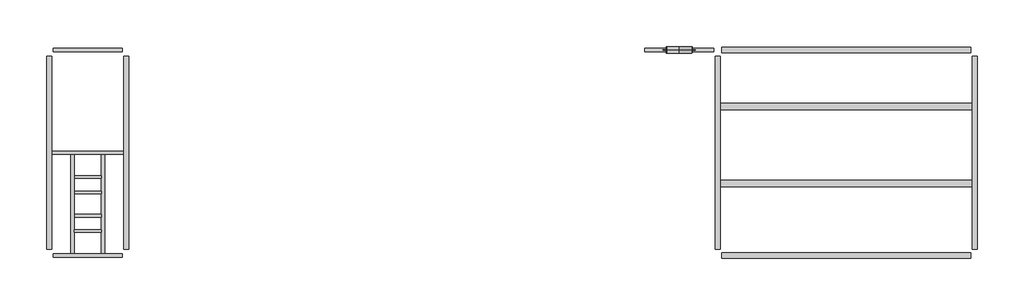
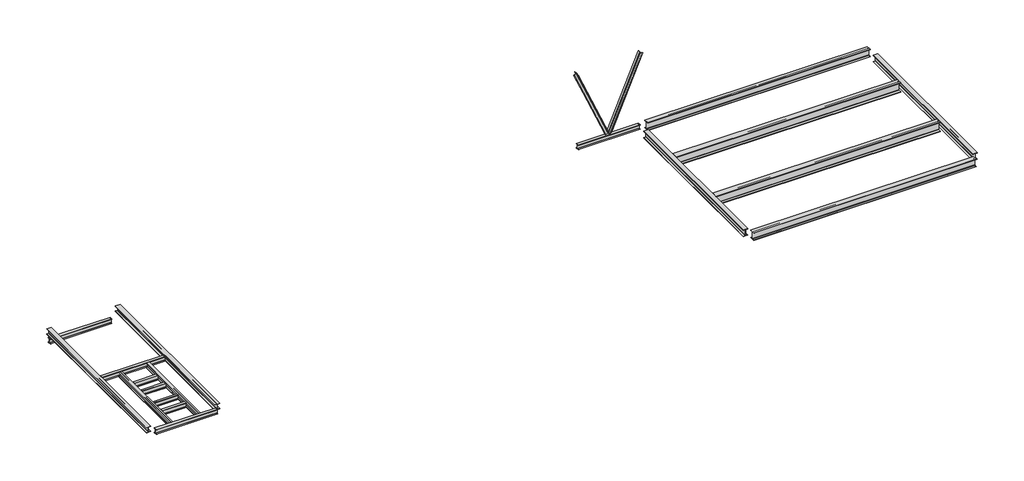
# One storey: 20 beams.
"""IFC4 building model written with IfcOpenShell, lengths in millimetres."""

import ifcopenshell
import ifcopenshell.guid

model = None  # the IFC model being written
_history = None  # IfcOwnerHistory: only IFC2X3 demands one
_inside = {}  # id of a spatial element -> (the spatial element, [elements in it])
_under = {}  # id of a project, library or spatial element -> (it, [spatial elements below it])
_declared = {}  # id of a project -> (the project, [libraries it declares])
_typed = {}  # id of a type object -> (the type object, [elements of that type])
_made_of = {}  # id of a material, layer set ... -> (it, [elements and type objects made of it])


def new_model(schema):
    """Start an empty IFC model of exactly this schema.

    Asked for "IFC4X3", IfcOpenShell would pick the latest addendum, in which some entities
    have other attributes; the version numbers below select the first issue.
    IFC2X3 requires an IfcOwnerHistory on every rooted entity: one is made here for all.
    """
    global model, _history
    if schema == "IFC4X3":
        model = ifcopenshell.file(schema_version=(4, 3, 0, 0))
    else:
        model = ifcopenshell.file(schema=schema)
    _inside.clear()
    _under.clear()
    _declared.clear()
    _typed.clear()
    _made_of.clear()
    _history = None
    if model.schema == "IFC2X3":
        org = make("IfcOrganization", Name="unknown")
        user = make(
            "IfcPersonAndOrganization",
            ThePerson=make("IfcPerson", FamilyName="unknown"),
            TheOrganization=org,
        )
        app = make(
            "IfcApplication",
            ApplicationDeveloper=org,
            Version="unknown",
            ApplicationFullName="unknown",
            ApplicationIdentifier="unknown",
        )
        _history = make(
            "IfcOwnerHistory",
            OwningUser=user,
            OwningApplication=app,
            ChangeAction="ADDED",
            CreationDate=0,
        )
    return model


def make(cls, **values):
    """One entity of the class cls with the attributes given. An attribute that is None is left unset."""
    return model.create_entity(
        cls, **{name: value for name, value in values.items() if value is not None}
    )


def rooted(cls, **values):
    """An entity with a GlobalId (a new one), such as an element, a storey or a relation."""
    return make(cls, GlobalId=ifcopenshell.guid.new(), OwnerHistory=_history, **values)


def si_unit(unit_type, name, prefix=None):
    """IfcSIUnit, for example si_unit("LENGTHUNIT", "METRE", prefix="MILLI")."""
    return make("IfcSIUnit", UnitType=unit_type, Prefix=prefix, Name=name)


def assignment(units):
    """IfcUnitAssignment: the units of a project."""
    return None if units is None else make("IfcUnitAssignment", Units=units)


def point(xyz):
    """IfcCartesianPoint."""
    return None if xyz is None else make("IfcCartesianPoint", Coordinates=xyz)


def direction(xyz):
    """IfcDirection."""
    return None if xyz is None else make("IfcDirection", DirectionRatios=xyz)


def frame(location, z_axis=None, x_axis=None):
    """IfcAxis2Placement3D, a coordinate frame: its origin and axes. An axis left out is left unset."""
    return make(
        "IfcAxis2Placement3D",
        Location=point(location),
        Axis=direction(z_axis),
        RefDirection=direction(x_axis),
    )


def frame_2d(location, x_axis=None):
    """IfcAxis2Placement2D, a coordinate frame in the plane: its origin and x axis."""
    return make(
        "IfcAxis2Placement2D", Location=point(location), RefDirection=direction(x_axis)
    )


def origin():
    """The frame at (0, 0, 0) with its axes left unset."""
    return frame((0.0, 0.0, 0.0))


def place(relative_to, where):
    """IfcLocalPlacement: puts the frame where relative to a parent placement (None: the world)."""
    return make(
        "IfcLocalPlacement", PlacementRelTo=relative_to, RelativePlacement=where
    )


def context(
    kind, dimensions, precision=None, world=None, true_north=None, identifier=None
):
    """IfcGeometricRepresentationContext, for example the 3D "Model" context."""
    return make(
        "IfcGeometricRepresentationContext",
        ContextIdentifier=identifier,
        ContextType=kind,
        CoordinateSpaceDimension=dimensions,
        Precision=precision,
        WorldCoordinateSystem=world,
        TrueNorth=true_north,
    )


def project(units=None, contexts=None):
    """IfcProject with its units and contexts."""
    return rooted(
        "IfcProject",
        Name="project",
        RepresentationContexts=contexts,
        UnitsInContext=assignment(units),
    )


def spatial(cls, under=None, at=None, **own):
    """A site, building, storey or space (cls), placed at a placement, below another one or the project."""
    s = rooted(cls, ObjectPlacement=at, **own)
    if under is not None:
        _under.setdefault(under.id(), (under, []))[1].append(s)
    return s


def polyline(points):
    """IfcPolyline through the points."""
    return make("IfcPolyline", Points=[point(p) for p in points])


def circle_curve(where, radius):
    """IfcCircle in the frame where."""
    return make("IfcCircle", Position=where, Radius=radius)


def trimmed(basis, trim1, trim2, sense, master):
    """IfcTrimmedCurve: the piece of a basis curve between two trims."""
    return make(
        "IfcTrimmedCurve",
        BasisCurve=basis,
        Trim1=trim1,
        Trim2=trim2,
        SenseAgreement=sense,
        MasterRepresentation=master,
    )


def segment(curve, same_sense, transition):
    """IfcCompositeCurveSegment."""
    return make(
        "IfcCompositeCurveSegment",
        Transition=transition,
        SameSense=same_sense,
        ParentCurve=curve,
    )


def composite_curve(segments, self_intersect=None):
    """IfcCompositeCurve: segments joined end to end."""
    return make("IfcCompositeCurve", Segments=segments, SelfIntersect=self_intersect)


def outline(outer, holes=None, kind="AREA"):
    """IfcArbitraryClosedProfileDef: a profile drawn as a closed curve; with holes, ...WithVoids."""
    if holes is None:
        return make("IfcArbitraryClosedProfileDef", ProfileType=kind, OuterCurve=outer)
    return make(
        "IfcArbitraryProfileDefWithVoids",
        ProfileType=kind,
        OuterCurve=outer,
        InnerCurves=holes,
    )


def extrude(swept, where, along, depth):
    """IfcExtrudedAreaSolid: the profile swept, set in the frame where, extruded along a direction by depth."""
    return make(
        "IfcExtrudedAreaSolid",
        SweptArea=swept,
        Position=where,
        ExtrudedDirection=direction(along),
        Depth=depth,
    )


def shape(context_of_items, identifier, shape_type, items):
    """IfcShapeRepresentation: the items that make up one representation, for example the "Body"."""
    return make(
        "IfcShapeRepresentation",
        ContextOfItems=context_of_items,
        RepresentationIdentifier=identifier,
        RepresentationType=shape_type,
        Items=items,
    )


def source(mapping_origin, context_of_items, identifier, shape_type, items):
    """IfcRepresentationMap: a shape defined once, which mapped items show again and again."""
    return make(
        "IfcRepresentationMap",
        MappingOrigin=mapping_origin,
        MappedRepresentation=shape(context_of_items, identifier, shape_type, items),
    )


def transform(
    local_origin,
    x_axis=None,
    y_axis=None,
    z_axis=None,
    scale=None,
    scale2=None,
    scale3=None,
    uniform=True,
):
    """IfcCartesianTransformationOperator3D, or its non-uniform kind. x_axis, y_axis, z_axis: its Axis1, 2, 3."""
    if uniform:
        return make(
            "IfcCartesianTransformationOperator3D",
            Axis1=direction(x_axis),
            Axis2=direction(y_axis),
            LocalOrigin=point(local_origin),
            Scale=scale,
            Axis3=direction(z_axis),
        )
    return make(
        "IfcCartesianTransformationOperator3DnonUniform",
        Axis1=direction(x_axis),
        Axis2=direction(y_axis),
        LocalOrigin=point(local_origin),
        Scale=scale,
        Axis3=direction(z_axis),
        Scale2=scale2,
        Scale3=scale3,
    )


def mapped(mapping_source, mapping_target):
    """IfcMappedItem: shows the shape of a source again, moved by a transform."""
    return make(
        "IfcMappedItem", MappingSource=mapping_source, MappingTarget=mapping_target
    )


def made_of(thing, what):
    """Note that an element or type object is made of a material, layer set ...; save() writes the relation."""
    if what is not None:
        _made_of.setdefault(what.id(), (what, []))[1].append(thing)
    return thing


def element(
    cls,
    number,
    at=None,
    inside=None,
    cuts=None,
    type_object=None,
    material=None,
    context=None,
    identifier="Body",
    shape_type=None,
    held_by="IfcProductDefinitionShape",
    body=None,
    shapes=None,
    **own,
):
    """One element of the class cls, such as IfcWall. Its Tag is "e" and its number.

    at: its placement. inside: the storey or other place that contains it. cuts: it is an
    opening in that element (IfcRelVoidsElement). A single representation is given by context,
    identifier, shape_type and body (its items); several are given by shapes. held_by: the class
    of the entity that holds the representations. save() writes the other relations.
    """
    e = rooted(cls, Tag="e%d" % number, ObjectPlacement=at, **own)
    if body is not None:
        shapes = [shape(context, identifier, shape_type, body)]
    if shapes is not None:
        e.Representation = make(held_by, Representations=shapes)
    if inside is not None:
        _inside.setdefault(inside.id(), (inside, []))[1].append(e)
    if cuts is not None:
        rooted(
            "IfcRelVoidsElement", RelatingBuildingElement=cuts, RelatedOpeningElement=e
        )
    if type_object is not None:
        _typed.setdefault(type_object.id(), (type_object, []))[1].append(e)
    return made_of(e, material)


def aggregate(whole, parts):
    """IfcRelAggregates: a whole, such as a stair, and the parts it consists of."""
    return rooted("IfcRelAggregates", RelatingObject=whole, RelatedObjects=parts)


def save(model, path):
    """Write the relations noted so far, then the file.

    IfcRelAggregates (storeys below a building ...), IfcRelContainedInSpatialStructure (elements
    in a storey), IfcRelDefinesByType, IfcRelAssociatesMaterial and IfcRelDeclares: one each for
    every whole, place, type object, material and project.
    """
    for whole, parts in _under.values():
        aggregate(whole, parts)
    for where, things in _inside.values():
        rooted(
            "IfcRelContainedInSpatialStructure",
            RelatedElements=things,
            RelatingStructure=where,
        )
    for kind, things in _typed.values():
        rooted("IfcRelDefinesByType", RelatedObjects=things, RelatingType=kind)
    for what, things in _made_of.values():
        rooted("IfcRelAssociatesMaterial", RelatedObjects=things, RelatingMaterial=what)
    for by, libraries in _declared.values():
        rooted("IfcRelDeclares", RelatingContext=by, RelatedDefinitions=libraries)
    model.write(path)


def beam_96e87236(model_context):
    return source(origin(), model_context, "Body", "SweptSolid", [
        extrude(outline(composite_curve([segment(polyline([(0.0, 36.4), (130.0, 36.4)]), True, "CONTINUOUS"), segment(trimmed(circle_curve(frame_2d((118.0, 36.4)), 12.0), [point((130.0, 36.4))], [point((118.0, 24.4))], False, "CARTESIAN"), True, "CONTINUOUS"), segment(polyline([(118.0, 24.4), (24.0, 24.4)]), True, "CONTINUOUS"), segment(trimmed(circle_curve(frame_2d((24.0, 12.4)), 12.0), [point((24.0, 24.4))], [point((12.0, 12.4))], True, "CARTESIAN"), True, "CONTINUOUS"), segment(polyline([(12.0, 12.4), (12.0, -81.6)]), True, "CONTINUOUS"), segment(trimmed(circle_curve(frame_2d((0.0, -81.6)), 12.0), [point((12.0, -81.6))], [point((0.0, -93.6))], False, "CARTESIAN"), True, "CONTINUOUS"), segment(polyline([(0.0, -93.6), (0.0, 36.4)]), True, "CONTINUOUS")], self_intersect=False)), frame((-1749.149537, 0.0, 0.0), z_axis=(1.0, 0.0, 0.0), x_axis=(0.0, 1.0, 0.0)), (0.0, 0.0, 1.0), 3498.299074),
        extrude(outline(composite_curve([segment(polyline([(0.0, 36.4), (0.0, -93.6)]), True, "CONTINUOUS"), segment(trimmed(circle_curve(frame_2d((0.0, -81.6)), 12.0), [point((0.0, -93.6))], [point((-12.0, -81.6))], False, "CARTESIAN"), True, "CONTINUOUS"), segment(polyline([(-12.0, -81.6), (-12.0, 12.4)]), True, "CONTINUOUS"), segment(trimmed(circle_curve(frame_2d((-24.0, 12.4)), 12.0), [point((-12.0, 12.4))], [point((-24.0, 24.4))], True, "CARTESIAN"), True, "CONTINUOUS"), segment(polyline([(-24.0, 24.4), (-118.0, 24.4)]), True, "CONTINUOUS"), segment(trimmed(circle_curve(frame_2d((-118.0, 36.4)), 12.0), [point((-118.0, 24.4))], [point((-130.0, 36.4))], False, "CARTESIAN"), True, "CONTINUOUS"), segment(polyline([(-130.0, 36.4), (0.0, 36.4)]), True, "CONTINUOUS")], self_intersect=False)), frame((-1749.149537, 0.0, 0.0), z_axis=(1.0, 0.0, 0.0), x_axis=(0.0, 1.0, 0.0)), (0.0, 0.0, 1.0), 3498.299074),
    ])


def steel_framing_w_astm_a6m_f33feb28(model_context):
    return source(origin(), model_context, "Body", "SweptSolid", [
        extrude(outline(composite_curve([segment(polyline([(67.0, -94.8), (67.0, -105.0), (-67.0, -105.0), (-67.0, -94.8), (-10.775, -94.8)]), True, "CONTINUOUS"), segment(trimmed(circle_curve(frame_2d((-10.775, -87.2)), 7.6), [point((-10.775, -94.8))], [point((-3.175, -87.2))], True, "CARTESIAN"), True, "CONTINUOUS"), segment(polyline([(-3.175, -87.2), (-3.175, 87.2)]), True, "CONTINUOUS"), segment(trimmed(circle_curve(frame_2d((-10.775, 87.2)), 7.6), [point((-3.175, 87.2))], [point((-10.775, 94.8))], True, "CARTESIAN"), True, "CONTINUOUS"), segment(polyline([(-10.775, 94.8), (-67.0, 94.8), (-67.0, 105.0), (67.0, 105.0), (67.0, 94.8), (10.775, 94.8)]), True, "CONTINUOUS"), segment(trimmed(circle_curve(frame_2d((10.775, 87.2)), 7.6), [point((10.775, 94.8))], [point((3.175, 87.2))], True, "CARTESIAN"), True, "CONTINUOUS"), segment(polyline([(3.175, 87.2), (3.175, -87.2)]), True, "CONTINUOUS"), segment(trimmed(circle_curve(frame_2d((10.775, -87.2)), 7.6), [point((3.175, -87.2))], [point((10.775, -94.8))], True, "CARTESIAN"), True, "CONTINUOUS"), segment(polyline([(10.775, -94.8), (67.0, -94.8)]), True, "CONTINUOUS")], self_intersect=False)), frame((-1346.3, 0.0, 0.0), z_axis=(1.0, 0.0, 0.0), x_axis=(0.0, 1.0, 0.0)), (0.0, 0.0, 1.0), 2692.6),
    ])


def steel_framing_w_astm_a6m_fe1e75f4(model_context):
    return source(origin(), model_context, "Body", "SweptSolid", [
        extrude(outline(composite_curve([segment(polyline([(67.0, -94.8), (67.0, -105.0), (-67.0, -105.0), (-67.0, -94.8), (-10.775, -94.8)]), True, "CONTINUOUS"), segment(trimmed(circle_curve(frame_2d((-10.775, -87.2)), 7.6), [point((-10.775, -94.8))], [point((-3.175, -87.2))], True, "CARTESIAN"), True, "CONTINUOUS"), segment(polyline([(-3.175, -87.2), (-3.175, 87.2)]), True, "CONTINUOUS"), segment(trimmed(circle_curve(frame_2d((-10.775, 87.2)), 7.6), [point((-3.175, 87.2))], [point((-10.775, 94.8))], True, "CARTESIAN"), True, "CONTINUOUS"), segment(polyline([(-10.775, 94.8), (-67.0, 94.8), (-67.0, 105.0), (67.0, 105.0), (67.0, 94.8), (10.775, 94.8)]), True, "CONTINUOUS"), segment(trimmed(circle_curve(frame_2d((10.775, 87.2)), 7.6), [point((10.775, 94.8))], [point((3.175, 87.2))], True, "CARTESIAN"), True, "CONTINUOUS"), segment(polyline([(3.175, 87.2), (3.175, -87.2)]), True, "CONTINUOUS"), segment(trimmed(circle_curve(frame_2d((10.775, -87.2)), 7.6), [point((3.175, -87.2))], [point((10.775, -94.8))], True, "CARTESIAN"), True, "CONTINUOUS"), segment(polyline([(10.775, -94.8), (67.0, -94.8)]), True, "CONTINUOUS")], self_intersect=False)), frame((-1386.3, 0.0, 0.0), z_axis=(1.0, 0.0, 0.0), x_axis=(0.0, 1.0, 0.0)), (0.0, 0.0, 1.0), 2772.6),
    ])


def steel_framing_w_astm_a6m_8cea9429(model_context):
    return source(origin(), model_context, "Body", "SweptSolid", [
        extrude(outline(composite_curve([segment(polyline([(101.5, -137.9), (101.5, -151.0), (-101.5, -151.0), (-101.5, -137.9), (-16.545, -137.9)]), True, "CONTINUOUS"), segment(trimmed(circle_curve(frame_2d((-16.545, -125.1)), 12.8), [point((-16.545, -137.9))], [point((-3.745, -125.1))], True, "CARTESIAN"), True, "CONTINUOUS"), segment(polyline([(-3.745, -125.1), (-3.745, 125.1)]), True, "CONTINUOUS"), segment(trimmed(circle_curve(frame_2d((-16.545, 125.1)), 12.8), [point((-3.745, 125.1))], [point((-16.545, 137.9))], True, "CARTESIAN"), True, "CONTINUOUS"), segment(polyline([(-16.545, 137.9), (-101.5, 137.9), (-101.5, 151.0), (101.5, 151.0), (101.5, 137.9), (16.545, 137.9)]), True, "CONTINUOUS"), segment(trimmed(circle_curve(frame_2d((16.545, 125.1)), 12.8), [point((16.545, 137.9))], [point((3.745, 125.1))], True, "CARTESIAN"), True, "CONTINUOUS"), segment(polyline([(3.745, 125.1), (3.745, -125.1)]), True, "CONTINUOUS"), segment(trimmed(circle_curve(frame_2d((16.545, -125.1)), 12.8), [point((3.745, -125.1))], [point((16.545, -137.9))], True, "CARTESIAN"), True, "CONTINUOUS"), segment(polyline([(16.545, -137.9), (101.5, -137.9)]), True, "CONTINUOUS")], self_intersect=False)), frame((-3753.8, 0.0, 0.0), z_axis=(1.0, 0.0, 0.0), x_axis=(0.0, 1.0, 0.0)), (0.0, 0.0, 1.0), 7507.6),
    ])


def steel_framing_w_astm_a6m_fd2852ff(model_context):
    return source(origin(), model_context, "Body", "SweptSolid", [
        extrude(outline(composite_curve([segment(polyline([(67.0, -94.8), (67.0, -105.0), (-67.0, -105.0), (-67.0, -94.8), (-10.775, -94.8)]), True, "CONTINUOUS"), segment(trimmed(circle_curve(frame_2d((-10.775, -87.2)), 7.6), [point((-10.775, -94.8))], [point((-3.175, -87.2))], True, "CARTESIAN"), True, "CONTINUOUS"), segment(polyline([(-3.175, -87.2), (-3.175, 87.2)]), True, "CONTINUOUS"), segment(trimmed(circle_curve(frame_2d((-10.775, 87.2)), 7.6), [point((-3.175, 87.2))], [point((-10.775, 94.8))], True, "CARTESIAN"), True, "CONTINUOUS"), segment(polyline([(-10.775, 94.8), (-67.0, 94.8), (-67.0, 105.0), (67.0, 105.0), (67.0, 94.8), (10.775, 94.8)]), True, "CONTINUOUS"), segment(trimmed(circle_curve(frame_2d((10.775, 87.2)), 7.6), [point((10.775, 94.8))], [point((3.175, 87.2))], True, "CARTESIAN"), True, "CONTINUOUS"), segment(polyline([(3.175, 87.2), (3.175, -87.2)]), True, "CONTINUOUS"), segment(trimmed(circle_curve(frame_2d((10.775, -87.2)), 7.6), [point((3.175, -87.2))], [point((10.775, -94.8))], True, "CARTESIAN"), True, "CONTINUOUS"), segment(polyline([(10.775, -94.8), (67.0, -94.8)]), True, "CONTINUOUS")], self_intersect=False)), frame((-1920.3, 0.0, 0.0), z_axis=(1.0, 0.0, 0.0), x_axis=(0.0, 1.0, 0.0)), (0.0, 0.0, 1.0), 3840.6),
    ])


def steel_framing_w_astm_a6m_80da07c9(model_context):
    return source(origin(), model_context, "Body", "SweptSolid", [
        extrude(outline(composite_curve([segment(polyline([(101.0, -112.5), (101.0, -123.5), (-101.0, -123.5), (-101.0, -112.5), (-16.385, -112.5)]), True, "CONTINUOUS"), segment(trimmed(circle_curve(frame_2d((-16.385, -99.8)), 12.7), [point((-16.385, -112.5))], [point((-3.685, -99.8))], True, "CARTESIAN"), True, "CONTINUOUS"), segment(polyline([(-3.685, -99.8), (-3.685, 99.8)]), True, "CONTINUOUS"), segment(trimmed(circle_curve(frame_2d((-16.385, 99.8)), 12.7), [point((-3.685, 99.8))], [point((-16.385, 112.5))], True, "CARTESIAN"), True, "CONTINUOUS"), segment(polyline([(-16.385, 112.5), (-101.0, 112.5), (-101.0, 123.5), (101.0, 123.5), (101.0, 112.5), (16.385, 112.5)]), True, "CONTINUOUS"), segment(trimmed(circle_curve(frame_2d((16.385, 99.8)), 12.7), [point((16.385, 112.5))], [point((3.685, 99.8))], True, "CARTESIAN"), True, "CONTINUOUS"), segment(polyline([(3.685, 99.8), (3.685, -99.8)]), True, "CONTINUOUS"), segment(trimmed(circle_curve(frame_2d((16.385, -99.8)), 12.7), [point((3.685, -99.8))], [point((16.385, -112.5))], True, "CARTESIAN"), True, "CONTINUOUS"), segment(polyline([(16.385, -112.5), (101.0, -112.5)]), True, "CONTINUOUS")], self_intersect=False)), frame((-3753.8, 0.0, 0.0), z_axis=(1.0, 0.0, 0.0), x_axis=(0.0, 1.0, 0.0)), (0.0, 0.0, 1.0), 7507.6),
    ])


def steel_framing_w_astm_a6m_d888c6d0(model_context):
    return source(origin(), model_context, "Body", "SweptSolid", [
        extrude(outline(composite_curve([segment(polyline([(102.5, -159.7), (102.5, -176.5), (-102.5, -176.5), (-102.5, -159.7), (-19.7, -159.7)]), True, "CONTINUOUS"), segment(trimmed(circle_curve(frame_2d((-19.7, -144.7)), 15.0), [point((-19.7, -159.7))], [point((-4.7, -144.7))], True, "CARTESIAN"), True, "CONTINUOUS"), segment(polyline([(-4.7, -144.7), (-4.7, 144.7)]), True, "CONTINUOUS"), segment(trimmed(circle_curve(frame_2d((-19.7, 144.7)), 15.0), [point((-4.7, 144.7))], [point((-19.7, 159.7))], True, "CARTESIAN"), True, "CONTINUOUS"), segment(polyline([(-19.7, 159.7), (-102.5, 159.7), (-102.5, 176.5), (102.5, 176.5), (102.5, 159.7), (19.7, 159.7)]), True, "CONTINUOUS"), segment(trimmed(circle_curve(frame_2d((19.7, 144.7)), 15.0), [point((19.7, 159.7))], [point((4.7, 144.7))], True, "CARTESIAN"), True, "CONTINUOUS"), segment(polyline([(4.7, 144.7), (4.7, -144.7)]), True, "CONTINUOUS"), segment(trimmed(circle_curve(frame_2d((19.7, -144.7)), 15.0), [point((4.7, -144.7))], [point((19.7, -159.7))], True, "CARTESIAN"), True, "CONTINUOUS"), segment(polyline([(19.7, -159.7), (102.5, -159.7)]), True, "CONTINUOUS")], self_intersect=False)), frame((-4846.3, 0.0, 0.0), z_axis=(1.0, 0.0, 0.0), x_axis=(0.0, 1.0, 0.0)), (0.0, 0.0, 1.0), 9692.6),
    ])


def steel_framing_w_astm_a6m_4c16a149(model_context):
    return source(origin(), model_context, "Body", "SweptSolid", [
        extrude(outline(composite_curve([segment(polyline([(131.0, -190.2), (131.0, -209.5), (-131.0, -209.5), (-131.0, -190.2), (-16.0, -190.2)]), True, "CONTINUOUS"), segment(trimmed(circle_curve(frame_2d((-16.0, -180.0)), 10.2), [point((-16.0, -190.2))], [point((-5.8, -180.0))], True, "CARTESIAN"), True, "CONTINUOUS"), segment(polyline([(-5.8, -180.0), (-5.8, 180.0)]), True, "CONTINUOUS"), segment(trimmed(circle_curve(frame_2d((-16.0, 180.0)), 10.2), [point((-5.8, 180.0))], [point((-16.0, 190.2))], True, "CARTESIAN"), True, "CONTINUOUS"), segment(polyline([(-16.0, 190.2), (-131.0, 190.2), (-131.0, 209.5), (131.0, 209.5), (131.0, 190.2), (16.0, 190.2)]), True, "CONTINUOUS"), segment(trimmed(circle_curve(frame_2d((16.0, 180.0)), 10.2), [point((16.0, 190.2))], [point((5.8, 180.0))], True, "CARTESIAN"), True, "CONTINUOUS"), segment(polyline([(5.8, 180.0), (5.8, -180.0)]), True, "CONTINUOUS"), segment(trimmed(circle_curve(frame_2d((16.0, -180.0)), 10.2), [point((5.8, -180.0))], [point((16.0, -190.2))], True, "CARTESIAN"), True, "CONTINUOUS"), segment(polyline([(16.0, -190.2), (131.0, -190.2)]), True, "CONTINUOUS")], self_intersect=False)), frame((-4885.8, 0.0, 0.0), z_axis=(1.0, 0.0, 0.0), x_axis=(0.0, 1.0, 0.0)), (0.0, 0.0, 1.0), 9771.6),
    ])


def steel_framing_w_astm_a6m_f88b2983(model_context):
    return source(origin(), model_context, "Body", "SweptSolid", [
        extrude(outline(composite_curve([segment(polyline([(51.0, -95.0), (51.0, -103.0), (-51.0, -103.0), (-51.0, -95.0), (-10.71, -95.0)]), True, "CONTINUOUS"), segment(trimmed(circle_curve(frame_2d((-10.71, -87.4)), 7.6), [point((-10.71, -95.0))], [point((-3.11, -87.4))], True, "CARTESIAN"), True, "CONTINUOUS"), segment(polyline([(-3.11, -87.4), (-3.11, 87.4)]), True, "CONTINUOUS"), segment(trimmed(circle_curve(frame_2d((-10.71, 87.4)), 7.6), [point((-3.11, 87.4))], [point((-10.71, 95.0))], True, "CARTESIAN"), True, "CONTINUOUS"), segment(polyline([(-10.71, 95.0), (-51.0, 95.0), (-51.0, 103.0), (51.0, 103.0), (51.0, 95.0), (10.71, 95.0)]), True, "CONTINUOUS"), segment(trimmed(circle_curve(frame_2d((10.71, 87.4)), 7.6), [point((10.71, 95.0))], [point((3.11, 87.4))], True, "CARTESIAN"), True, "CONTINUOUS"), segment(polyline([(3.11, 87.4), (3.11, -87.4)]), True, "CONTINUOUS"), segment(trimmed(circle_curve(frame_2d((10.71, -87.4)), 7.6), [point((3.11, -87.4))], [point((10.71, -95.0))], True, "CARTESIAN"), True, "CONTINUOUS"), segment(polyline([(10.71, -95.0), (51.0, -95.0)]), True, "CONTINUOUS")], self_intersect=False)), frame((-520.3, 0.0, 0.0), z_axis=(1.0, 0.0, 0.0), x_axis=(0.0, 1.0, 0.0)), (0.0, 0.0, 1.0), 1040.6),
    ])


model = new_model("IFC4")

# Units and contexts
model_context = context("Model", 3, world=origin())
ifc_project = project(units=[si_unit("LENGTHUNIT", "METRE", prefix="MILLI")], contexts=[model_context])

# Site, building, storey
site = spatial("IfcSite", under=ifc_project)
building = spatial("IfcBuilding", under=site)
storey = spatial("IfcBuildingStorey", under=building, Name="T.O.S(4)", Elevation=5219.8243501)

# Beams
placement = place(None, origin())
beam_shape = beam_96e87236(model_context)
element("IfcBeam", 1, ObjectType="0123_Steel Framing_2Ls-KSD3502 : H_SB_AR_S04_2Ls-130x130x12_VBR1", at=placement, inside=storey, context=model_context, shape_type="MappedRepresentation", body=[
    mapped(beam_shape, transform((25223.7124521, 22499.5208589, 6876.090442), x_axis=(0.39391929857916597, 0.0, 0.9191450300180586), y_axis=(0.0, 1.0, 0.0), z_axis=(-0.9191450300180586, 0.0, 0.39391929857916597))),
])
element("IfcBeam", 2, ObjectType="0123_Steel Framing_2Ls-KSD3502 : H_SB_AR_S04_2Ls-130x130x12_VBR1", at=placement, inside=storey, context=model_context, shape_type="MappedRepresentation", body=[
    mapped(beam_shape, transform((23776.2875479, 22499.5208589, 6876.090442), x_axis=(0.3939192985791688, 0.0, -0.9191450300180575), y_axis=(0.0, 1.0, 0.0), z_axis=(0.9191450300180575, 0.0, 0.3939192985791688))),
])
steel_framing_w_astm_a6m_shape = steel_framing_w_astm_a6m_f33feb28(model_context)
element("IfcBeam", 3, ObjectType="Steel Framing_W_ASTM A6M : H_SB_AR_S02_W200x31.3_B6", at=placement, inside=storey, context=model_context, shape_type="MappedRepresentation", body=[
    mapped(steel_framing_w_astm_a6m_shape, transform((1500.0, 22499.5208589, 4214.8243501), x_axis=(1.0, 0.0, 0.0), y_axis=(0.0, 1.0, 0.0), z_axis=(0.0, 0.0, 1.0))),
])
element("IfcBeam", 4, ObjectType="Steel Framing_W_ASTM A6M : H_SB_AR_S02_W200x31.3_B6", at=placement, inside=storey, context=model_context, shape_type="MappedRepresentation", body=[
    mapped(steel_framing_w_astm_a6m_shape, transform((1500.0, 14499.5208589, 4899.8243501), x_axis=(1.0, 0.0, 0.0), y_axis=(0.0, 1.0, 0.0), z_axis=(0.0, 0.0, 1.0))),
])
element("IfcBeam", 5, ObjectType="Steel Framing_W_ASTM A6M : H_SB_AR_S02_W200x31.3_B6", at=placement, inside=storey, context=model_context, shape_type="MappedRepresentation", body=[
    mapped(steel_framing_w_astm_a6m_shape, transform((24500.0, 22499.5208589, 5114.8243501), x_axis=(1.0, 0.0, 0.0), y_axis=(0.0, 1.0, 0.0), z_axis=(0.0, 0.0, 1.0))),
])
steel_framing_w_astm_a6m_2_shape = steel_framing_w_astm_a6m_fe1e75f4(model_context)
element("IfcBeam", 6, ObjectType="Steel Framing_W_ASTM A6M : H_SB_AR_S02_W200x31.3_B6", at=placement, inside=storey, context=model_context, shape_type="MappedRepresentation", body=[
    mapped(steel_framing_w_astm_a6m_2_shape, transform((1500.0, 18499.5208589, 4899.8243501), x_axis=(1.0, 0.0, 0.0), y_axis=(0.0, 1.0, 0.0), z_axis=(0.0, 0.0, 1.0))),
])
steel_framing_w_astm_a6m_3_shape = steel_framing_w_astm_a6m_8cea9429(model_context)
element("IfcBeam", 7, ObjectType="Steel Framing_W_ASTM A6M : H_SB_AR_S02_W310x60_G4", at=placement, inside=storey, context=model_context, shape_type="MappedRepresentation", body=[
    mapped(steel_framing_w_astm_a6m_3_shape, transform((26000.0, 18499.5208589, 4853.8243501), x_axis=(0.0, 1.0, 0.0), y_axis=(-1.0, 0.0, 0.0), z_axis=(0.0, 0.0, 1.0))),
])
element("IfcBeam", 8, ObjectType="Steel Framing_W_ASTM A6M : H_SB_AR_S02_W310x60_G4", at=placement, inside=storey, context=model_context, shape_type="MappedRepresentation", body=[
    mapped(steel_framing_w_astm_a6m_3_shape, transform((36000.0, 18499.5208589, 4853.8243501), x_axis=(0.0, 1.0, 0.0), y_axis=(-1.0, 0.0, 0.0), z_axis=(0.0, 0.0, 1.0))),
])
steel_framing_w_astm_a6m_4_shape = steel_framing_w_astm_a6m_fd2852ff(model_context)
element("IfcBeam", 9, ObjectType="Steel Framing_W_ASTM A6M : H_SB_AR_S02_W200x31.3_B6", at=placement, inside=storey, context=model_context, shape_type="MappedRepresentation", body=[
    mapped(steel_framing_w_astm_a6m_4_shape, transform((900.0, 16499.5208589, 4899.8243501), x_axis=(0.0, -1.0, 0.0), y_axis=(1.0, 0.0, 0.0), z_axis=(0.0, 0.0, 1.0))),
])
element("IfcBeam", 10, ObjectType="Steel Framing_W_ASTM A6M : H_SB_AR_S02_W200x31.3_B6", at=placement, inside=storey, context=model_context, shape_type="MappedRepresentation", body=[
    mapped(steel_framing_w_astm_a6m_4_shape, transform((2100.0, 16499.5208589, 4899.8243501), x_axis=(0.0, -1.0, 0.0), y_axis=(1.0, 0.0, 0.0), z_axis=(0.0, 0.0, 1.0))),
])
steel_framing_w_astm_a6m_5_shape = steel_framing_w_astm_a6m_80da07c9(model_context)
element("IfcBeam", 11, ObjectType="Steel Framing_W_ASTM A6M : H_SB_AR_S02_W250x49.1_G5", at=placement, inside=storey, context=model_context, shape_type="MappedRepresentation", body=[
    mapped(steel_framing_w_astm_a6m_5_shape, transform((0.0, 18499.5208589, 4881.3243501), x_axis=(0.0, 1.0, 0.0), y_axis=(-1.0, 0.0, 0.0), z_axis=(0.0, 0.0, 1.0))),
])
element("IfcBeam", 12, ObjectType="Steel Framing_W_ASTM A6M : H_SB_AR_S02_W250x49.1_G5", at=placement, inside=storey, context=model_context, shape_type="MappedRepresentation", body=[
    mapped(steel_framing_w_astm_a6m_5_shape, transform((3000.0, 18499.5208589, 4881.3243501), x_axis=(0.0, -1.0, 0.0), y_axis=(1.0, 0.0, 0.0), z_axis=(0.0, 0.0, 1.0))),
])
steel_framing_w_astm_a6m_6_shape = steel_framing_w_astm_a6m_d888c6d0(model_context)
element("IfcBeam", 13, ObjectType="Steel Framing_W_ASTM A6M : H_SB_AR_S02_W360x79_B2", at=placement, inside=storey, context=model_context, shape_type="MappedRepresentation", body=[
    mapped(steel_framing_w_astm_a6m_6_shape, transform((31000.0, 22499.5208589, 5043.3243501), x_axis=(1.0, 0.0, 0.0), y_axis=(0.0, 1.0, 0.0), z_axis=(0.0, 0.0, 1.0))),
])
element("IfcBeam", 14, ObjectType="Steel Framing_W_ASTM A6M : H_SB_AR_S02_W360x79_B2", at=placement, inside=storey, context=model_context, shape_type="MappedRepresentation", body=[
    mapped(steel_framing_w_astm_a6m_6_shape, transform((31000.0, 14499.5208589, 4828.3243501), x_axis=(1.0, 0.0, 0.0), y_axis=(0.0, 1.0, 0.0), z_axis=(0.0, 0.0, 1.0))),
])
steel_framing_w_astm_a6m_7_shape = steel_framing_w_astm_a6m_4c16a149(model_context)
element("IfcBeam", 15, ObjectType="Steel Framing_W_ASTM A6M : H_SB_AR_S02_W410x114_B9", at=placement, inside=storey, context=model_context, shape_type="MappedRepresentation", body=[
    mapped(steel_framing_w_astm_a6m_7_shape, transform((31000.0, 20299.5208589, 4795.3243501), x_axis=(1.0, 0.0, 0.0), y_axis=(0.0, 1.0, 0.0), z_axis=(0.0, 0.0, 1.0))),
])
element("IfcBeam", 16, ObjectType="Steel Framing_W_ASTM A6M : H_SB_AR_S02_W410x114_B9", at=placement, inside=storey, context=model_context, shape_type="MappedRepresentation", body=[
    mapped(steel_framing_w_astm_a6m_7_shape, transform((31000.0, 17299.5208589, 4795.3243501), x_axis=(1.0, 0.0, 0.0), y_axis=(0.0, 1.0, 0.0), z_axis=(0.0, 0.0, 1.0))),
])
steel_framing_w_astm_a6m_8_shape = steel_framing_w_astm_a6m_f88b2983(model_context)
element("IfcBeam", 17, ObjectType="Steel Framing_W_ASTM A6M : H_SB_AR_S02_W200x22.5_J1", at=placement, inside=storey, context=model_context, shape_type="MappedRepresentation", body=[
    mapped(steel_framing_w_astm_a6m_8_shape, transform((1500.0, 17549.5208589, 4901.8243501), x_axis=(1.0, 0.0, 0.0), y_axis=(0.0, 1.0, 0.0), z_axis=(0.0, 0.0, 1.0))),
])
element("IfcBeam", 18, ObjectType="Steel Framing_W_ASTM A6M : H_SB_AR_S02_W200x22.5_J1", at=placement, inside=storey, context=model_context, shape_type="MappedRepresentation", body=[
    mapped(steel_framing_w_astm_a6m_8_shape, transform((1500.0, 16949.5208589, 4901.8243501), x_axis=(1.0, 0.0, 0.0), y_axis=(0.0, 1.0, 0.0), z_axis=(0.0, 0.0, 1.0))),
])
element("IfcBeam", 19, ObjectType="Steel Framing_W_ASTM A6M : H_SB_AR_S02_W200x22.5_J1", at=placement, inside=storey, context=model_context, shape_type="MappedRepresentation", body=[
    mapped(steel_framing_w_astm_a6m_8_shape, transform((1500.0, 16049.5208589, 4901.8243501), x_axis=(1.0, 0.0, 0.0), y_axis=(0.0, 1.0, 0.0), z_axis=(0.0, 0.0, 1.0))),
])
element("IfcBeam", 20, ObjectType="Steel Framing_W_ASTM A6M : H_SB_AR_S02_W200x22.5_J1", at=placement, inside=storey, context=model_context, shape_type="MappedRepresentation", body=[
    mapped(steel_framing_w_astm_a6m_8_shape, transform((1500.0, 15449.5208589, 4901.8243501), x_axis=(1.0, 0.0, 0.0), y_axis=(0.0, 1.0, 0.0), z_axis=(0.0, 0.0, 1.0))),
])

save(model, "model.ifc")

# Revit data of these elements
# Type "0123_Steel Framing_2Ls-KSD3502 : H_SB_AR_S04_2Ls-130x130x12_VBR1"
#   Type Mark = "VBR1"
#   Assembly Code = "B10"
#   Legs = "SLBB"
#   W = 8.97
#   Perimeter = 1.04 m²/m
#   Nominal Weight = 46.80 kgf/m
#   Length [instance default] = 1000 mm
#   Space = 0 mm
#   b = 130 mm
#   d = 130 mm
#   t = 12 mm
#   y = 36.4 mm
#   A = 0.005952 m²
#   Structural Material [instance default] = Steel ASTM A36
# Type "Steel Framing_W_ASTM A6M : H_SB_AR_S02_W200x31.3_B6"
#   Type Mark = "B6"
#   Section Name Key = "W8x21"
#   Width = 13.4 cm
#   Web Thickness = 0.635 cm
#   Web Fillet = 0.76 cm
#   Warping Constant = 40800.0 cm⁶
#   Torsional Moment of Inertia = 11.70 cm⁴
#   Section Area = 39.7 cm²
#   Plastic Modulus weak axis = 93.2 cm³
#   Plastic Modulus strong axis = 334.0 cm³
#   Perimeter = 0.93 m²/m
#   Nominal Weight = 31.30 kgf/m
#   Moment of Inertia weak axis = 407.00 cm⁴
#   Moment of Inertia strong axis = 3130.00 cm⁴
#   Height = 21.0 cm
#   Flange Thickness = 1.02 cm
#   Elastic Modulus weak axis = 60.8 cm³
#   Elastic Modulus strong axis = 298.0 cm³
#   Centroid Vertical = 10.5 cm
#   Centroid Horizontal = 6.7 cm
#   Length [instance default] = 1500 mm
#   Structural Material [instance default] = Steel, 45-345
#   Bolt Spacing = 0
#   Assembly Code = ""
# Type "Steel Framing_W_ASTM A6M : H_SB_AR_S02_W310x60_G4"
#   Type Mark = "G4"
#   Section Name Key = "W12x40"
#   Width = 20.3 cm
#   Web Thickness = 0.749 cm
#   Web Fillet = 1.28 cm
#   Warping Constant = 387000.0 cm⁶
#   Torsional Moment of Inertia = 37.70 cm⁴
#   Section Area = 75.5 cm²
#   Plastic Modulus weak axis = 275.0 cm³
#   Plastic Modulus strong axis = 934.0 cm³
#   Perimeter = 1.38 m²/m
#   Nominal Weight = 60.00 kgf/m
#   Moment of Inertia weak axis = 1840.00 cm⁴
#   Moment of Inertia strong axis = 12800.00 cm⁴
#   Height = 30.2 cm
#   Flange Thickness = 1.31 cm
#   Elastic Modulus weak axis = 180.0 cm³
#   Elastic Modulus strong axis = 844.0 cm³
#   Centroid Vertical = 15.1 cm
#   Centroid Horizontal = 10.15 cm
#   Length [instance default] = 1500 mm
#   Structural Material [instance default] = Steel, 45-345
#   Bolt Spacing = 0
#   Assembly Code = ""
# Type "Steel Framing_W_ASTM A6M : H_SB_AR_S02_W250x49.1_G5"
#   Type Mark = "G5"
#   Section Name Key = "W10x33"
#   Width = 20.2 cm
#   Web Thickness = 0.737 cm
#   Web Fillet = 1.27 cm
#   Warping Constant = 212000.0 cm⁶
#   Torsional Moment of Inertia = 24.30 cm⁴
#   Section Area = 62.6 cm²
#   Plastic Modulus weak axis = 229.0 cm³
#   Plastic Modulus strong axis = 636.0 cm³
#   Perimeter = 1.27 m²/m
#   Nominal Weight = 49.10 kgf/m
#   Moment of Inertia weak axis = 1520.00 cm⁴
#   Moment of Inertia strong axis = 7120.00 cm⁴
#   Height = 24.7 cm
#   Flange Thickness = 1.1 cm
#   Elastic Modulus weak axis = 151.0 cm³
#   Elastic Modulus strong axis = 574.0 cm³
#   Centroid Vertical = 12.35 cm
#   Centroid Horizontal = 10.1 cm
#   Length [instance default] = 1500 mm
#   Structural Material [instance default] = Steel, 45-345
#   Bolt Spacing = 0
#   Assembly Code = ""
# Type "Steel Framing_W_ASTM A6M : H_SB_AR_S02_W360x79_B2"
#   Section Name Key = "W14x53"
#   Width = 20.5 cm
#   Web Thickness = 0.94 cm
#   Web Fillet = 1.5 cm
#   Warping Constant = 682000.0 cm⁶
#   Torsional Moment of Inertia = 80.70 cm⁴
#   Section Area = 101.0 cm²
#   Plastic Modulus weak axis = 361.0 cm³
#   Plastic Modulus strong axis = 1430.0 cm³
#   Perimeter = 1.48 m²/m
#   Nominal Weight = 79.00 kgf/m
#   Moment of Inertia weak axis = 2400.00 cm⁴
#   Moment of Inertia strong axis = 22500.00 cm⁴
#   Height = 35.3 cm
#   Flange Thickness = 1.68 cm
#   Elastic Modulus weak axis = 234.0 cm³
#   Elastic Modulus strong axis = 1270.0 cm³
#   Centroid Vertical = 17.65 cm
#   Centroid Horizontal = 10.25 cm
#   Length [instance default] = 1500 mm
#   Structural Material [instance default] = Steel, 45-345
#   Bolt Spacing = 0
#   Assembly Code = ""
# Type "Steel Framing_W_ASTM A6M : H_SB_AR_S02_W410x114_B9"
#   Section Name Key = "W16x77"
#   Width = 26.2 cm
#   Web Thickness = 1.16 cm
#   Web Fillet = 1.02 cm
#   Warping Constant = 2310000.0 cm⁶
#   Torsional Moment of Inertia = 149.00 cm⁴
#   Section Area = 146.0 cm²
#   Plastic Modulus weak axis = 674.0 cm³
#   Plastic Modulus strong axis = 2460.0 cm³
#   Perimeter = 1.84 m²/m
#   Nominal Weight = 114.00 kgf/m
#   Moment of Inertia weak axis = 5740.00 cm⁴
#   Moment of Inertia strong axis = 46200.00 cm⁴
#   Height = 41.9 cm
#   Flange Thickness = 1.93 cm
#   Elastic Modulus weak axis = 441.0 cm³
#   Elastic Modulus strong axis = 2200.0 cm³
#   Centroid Vertical = 20.95 cm
#   Centroid Horizontal = 13.1 cm
#   Length [instance default] = 1500 mm
#   Structural Material [instance default] = Steel, 45-345
#   Bolt Spacing = 0
#   Assembly Code = ""
# Type "Steel Framing_W_ASTM A6M : H_SB_AR_S02_W200x22.5_J1"
#   Section Name Key = "W8x15"
#   Width = 10.2 cm
#   Web Thickness = 0.622 cm
#   Web Fillet = 0.76 cm
#   Warping Constant = 13900.0 cm⁶
#   Torsional Moment of Inertia = 5.70 cm⁴
#   Section Area = 28.6 cm²
#   Plastic Modulus weak axis = 43.8 cm³
#   Plastic Modulus strong axis = 223.0 cm³
#   Perimeter = 0.795 m²/m
#   Nominal Weight = 22.50 kgf/m
#   Moment of Inertia weak axis = 142.00 cm⁴
#   Moment of Inertia strong axis = 2000.00 cm⁴
#   Height = 20.6 cm
#   Flange Thickness = 0.8 cm
#   Elastic Modulus weak axis = 27.9 cm³
#   Elastic Modulus strong axis = 193.0 cm³
#   Centroid Vertical = 10.3 cm
#   Centroid Horizontal = 5.1 cm
#   Length [instance default] = 1500 mm
#   Structural Material [instance default] = Steel, 45-345
#   Bolt Spacing = 0
#   Assembly Code = ""
# Elements 1, 2 (IfcBeam, "0123_Steel Framing_2Ls-KSD3502 : H_SB_AR_S04_2Ls-130x130x12_VBR1")
#   Structural Material = Steel ASTM A36
#   Phase Created = New Construction
#   Materials on its faces: "Steel ASTM A36"
# Elements 3, 4, 5, 6, 9, 10 (IfcBeam, "Steel Framing_W_ASTM A6M : H_SB_AR_S02_W200x31.3_B6")
#   Structural Material = Steel, 45-345
#   Phase Created = New Construction
#   Materials on its faces: "Steel, 45-345"
# Elements 7, 8 (IfcBeam, "Steel Framing_W_ASTM A6M : H_SB_AR_S02_W310x60_G4")
#   Structural Material = Steel, 45-345
#   Phase Created = New Construction
#   Materials on its faces: "Steel, 45-345"
# Elements 11, 12 (IfcBeam, "Steel Framing_W_ASTM A6M : H_SB_AR_S02_W250x49.1_G5")
#   Structural Material = Steel, 45-345
#   Phase Created = New Construction
#   Materials on its faces: "Steel, 45-345"
# Elements 13, 14 (IfcBeam, "Steel Framing_W_ASTM A6M : H_SB_AR_S02_W360x79_B2")
#   Structural Material = Steel, 45-345
#   Phase Created = New Construction
#   Materials on its faces: "Steel, 45-345"
# Elements 15, 16 (IfcBeam, "Steel Framing_W_ASTM A6M : H_SB_AR_S02_W410x114_B9")
#   Structural Material = Steel, 45-345
#   Phase Created = New Construction
#   Materials on its faces: "Steel, 45-345"
# Elements 17, 18, 19, 20 (IfcBeam, "Steel Framing_W_ASTM A6M : H_SB_AR_S02_W200x22.5_J1")
#   Structural Material = Steel ASTM A36
#   Phase Created = New Construction
#   Materials on its faces: "Steel ASTM A36"
# Materials
#   "Steel ASTM A36": class "Metal", colour RGB 199 199 199, transparency 0, Description = "Structural steel, ASTM A36 Grade B, mill finish", Cost = 0
#   "Steel, 45-345": class "Metal", colour RGB 189 187 185, transparency 0, Description = "Steel 345 MPa", Cost = 0
